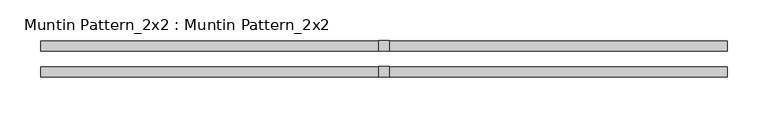
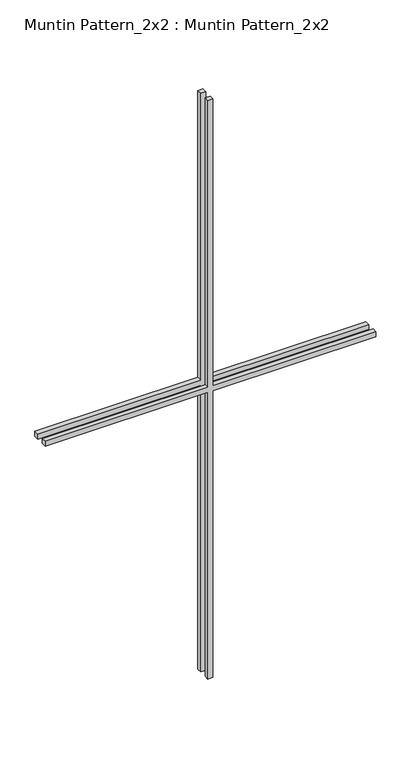
"""IFC4 building model written with IfcOpenShell, lengths in millimetres: proxy geometry, Muntin Pattern_2x2 : Muntin Pattern_2x2."""

import ifcopenshell
import ifcopenshell.guid

model = None  # the IFC model being written
_history = None  # IfcOwnerHistory: only IFC2X3 demands one
_inside = {}  # id of a spatial element -> (the spatial element, [elements in it])
_under = {}  # id of a project, library or spatial element -> (it, [spatial elements below it])
_declared = {}  # id of a project -> (the project, [libraries it declares])
_typed = {}  # id of a type object -> (the type object, [elements of that type])
_made_of = {}  # id of a material, layer set ... -> (it, [elements and type objects made of it])


def new_model(schema):
    """Start an empty IFC model of exactly this schema.

    Asked for "IFC4X3", IfcOpenShell would pick the latest addendum, in which some entities
    have other attributes; the version numbers below select the first issue.
    IFC2X3 requires an IfcOwnerHistory on every rooted entity: one is made here for all.
    """
    global model, _history
    if schema == "IFC4X3":
        model = ifcopenshell.file(schema_version=(4, 3, 0, 0))
    else:
        model = ifcopenshell.file(schema=schema)
    _inside.clear()
    _under.clear()
    _declared.clear()
    _typed.clear()
    _made_of.clear()
    _history = None
    if model.schema == "IFC2X3":
        org = make("IfcOrganization", Name="unknown")
        user = make(
            "IfcPersonAndOrganization",
            ThePerson=make("IfcPerson", FamilyName="unknown"),
            TheOrganization=org,
        )
        app = make(
            "IfcApplication",
            ApplicationDeveloper=org,
            Version="unknown",
            ApplicationFullName="unknown",
            ApplicationIdentifier="unknown",
        )
        _history = make(
            "IfcOwnerHistory",
            OwningUser=user,
            OwningApplication=app,
            ChangeAction="ADDED",
            CreationDate=0,
        )
    return model


def make(cls, **values):
    """One entity of the class cls with the attributes given. An attribute that is None is left unset."""
    return model.create_entity(
        cls, **{name: value for name, value in values.items() if value is not None}
    )


def rooted(cls, **values):
    """An entity with a GlobalId (a new one), such as an element, a storey or a relation."""
    return make(cls, GlobalId=ifcopenshell.guid.new(), OwnerHistory=_history, **values)


def si_unit(unit_type, name, prefix=None):
    """IfcSIUnit, for example si_unit("LENGTHUNIT", "METRE", prefix="MILLI")."""
    return make("IfcSIUnit", UnitType=unit_type, Prefix=prefix, Name=name)


def assignment(units):
    """IfcUnitAssignment: the units of a project."""
    return None if units is None else make("IfcUnitAssignment", Units=units)


def point(xyz):
    """IfcCartesianPoint."""
    return None if xyz is None else make("IfcCartesianPoint", Coordinates=xyz)


def direction(xyz):
    """IfcDirection."""
    return None if xyz is None else make("IfcDirection", DirectionRatios=xyz)


def frame(location, z_axis=None, x_axis=None):
    """IfcAxis2Placement3D, a coordinate frame: its origin and axes. An axis left out is left unset."""
    return make(
        "IfcAxis2Placement3D",
        Location=point(location),
        Axis=direction(z_axis),
        RefDirection=direction(x_axis),
    )


def origin():
    """The frame at (0, 0, 0) with its axes left unset."""
    return frame((0.0, 0.0, 0.0))


def place(relative_to, where):
    """IfcLocalPlacement: puts the frame where relative to a parent placement (None: the world)."""
    return make(
        "IfcLocalPlacement", PlacementRelTo=relative_to, RelativePlacement=where
    )


def context(
    kind, dimensions, precision=None, world=None, true_north=None, identifier=None
):
    """IfcGeometricRepresentationContext, for example the 3D "Model" context."""
    return make(
        "IfcGeometricRepresentationContext",
        ContextIdentifier=identifier,
        ContextType=kind,
        CoordinateSpaceDimension=dimensions,
        Precision=precision,
        WorldCoordinateSystem=world,
        TrueNorth=true_north,
    )


def project(units=None, contexts=None):
    """IfcProject with its units and contexts."""
    return rooted(
        "IfcProject",
        Name="project",
        RepresentationContexts=contexts,
        UnitsInContext=assignment(units),
    )


def spatial(cls, under=None, at=None, **own):
    """A site, building, storey or space (cls), placed at a placement, below another one or the project."""
    s = rooted(cls, ObjectPlacement=at, **own)
    if under is not None:
        _under.setdefault(under.id(), (under, []))[1].append(s)
    return s


def polyline(points):
    """IfcPolyline through the points."""
    return make("IfcPolyline", Points=[point(p) for p in points])


def outline(outer, holes=None, kind="AREA"):
    """IfcArbitraryClosedProfileDef: a profile drawn as a closed curve; with holes, ...WithVoids."""
    if holes is None:
        return make("IfcArbitraryClosedProfileDef", ProfileType=kind, OuterCurve=outer)
    return make(
        "IfcArbitraryProfileDefWithVoids",
        ProfileType=kind,
        OuterCurve=outer,
        InnerCurves=holes,
    )


def extrude(swept, where, along, depth):
    """IfcExtrudedAreaSolid: the profile swept, set in the frame where, extruded along a direction by depth."""
    return make(
        "IfcExtrudedAreaSolid",
        SweptArea=swept,
        Position=where,
        ExtrudedDirection=direction(along),
        Depth=depth,
    )


def shape(context_of_items, identifier, shape_type, items):
    """IfcShapeRepresentation: the items that make up one representation, for example the "Body"."""
    return make(
        "IfcShapeRepresentation",
        ContextOfItems=context_of_items,
        RepresentationIdentifier=identifier,
        RepresentationType=shape_type,
        Items=items,
    )


def source(mapping_origin, context_of_items, identifier, shape_type, items):
    """IfcRepresentationMap: a shape defined once, which mapped items show again and again."""
    return make(
        "IfcRepresentationMap",
        MappingOrigin=mapping_origin,
        MappedRepresentation=shape(context_of_items, identifier, shape_type, items),
    )


def transform(
    local_origin,
    x_axis=None,
    y_axis=None,
    z_axis=None,
    scale=None,
    scale2=None,
    scale3=None,
    uniform=True,
):
    """IfcCartesianTransformationOperator3D, or its non-uniform kind. x_axis, y_axis, z_axis: its Axis1, 2, 3."""
    if uniform:
        return make(
            "IfcCartesianTransformationOperator3D",
            Axis1=direction(x_axis),
            Axis2=direction(y_axis),
            LocalOrigin=point(local_origin),
            Scale=scale,
            Axis3=direction(z_axis),
        )
    return make(
        "IfcCartesianTransformationOperator3DnonUniform",
        Axis1=direction(x_axis),
        Axis2=direction(y_axis),
        LocalOrigin=point(local_origin),
        Scale=scale,
        Axis3=direction(z_axis),
        Scale2=scale2,
        Scale3=scale3,
    )


def mapped(mapping_source, mapping_target):
    """IfcMappedItem: shows the shape of a source again, moved by a transform."""
    return make(
        "IfcMappedItem", MappingSource=mapping_source, MappingTarget=mapping_target
    )


def made_of(thing, what):
    """Note that an element or type object is made of a material, layer set ...; save() writes the relation."""
    if what is not None:
        _made_of.setdefault(what.id(), (what, []))[1].append(thing)
    return thing


def element(
    cls,
    number,
    at=None,
    inside=None,
    cuts=None,
    type_object=None,
    material=None,
    context=None,
    identifier="Body",
    shape_type=None,
    held_by="IfcProductDefinitionShape",
    body=None,
    shapes=None,
    **own,
):
    """One element of the class cls, such as IfcWall. Its Tag is "e" and its number.

    at: its placement. inside: the storey or other place that contains it. cuts: it is an
    opening in that element (IfcRelVoidsElement). A single representation is given by context,
    identifier, shape_type and body (its items); several are given by shapes. held_by: the class
    of the entity that holds the representations. save() writes the other relations.
    """
    e = rooted(cls, Tag="e%d" % number, ObjectPlacement=at, **own)
    if body is not None:
        shapes = [shape(context, identifier, shape_type, body)]
    if shapes is not None:
        e.Representation = make(held_by, Representations=shapes)
    if inside is not None:
        _inside.setdefault(inside.id(), (inside, []))[1].append(e)
    if cuts is not None:
        rooted(
            "IfcRelVoidsElement", RelatingBuildingElement=cuts, RelatedOpeningElement=e
        )
    if type_object is not None:
        _typed.setdefault(type_object.id(), (type_object, []))[1].append(e)
    return made_of(e, material)


def aggregate(whole, parts):
    """IfcRelAggregates: a whole, such as a stair, and the parts it consists of."""
    return rooted("IfcRelAggregates", RelatingObject=whole, RelatedObjects=parts)


def save(model, path):
    """Write the relations noted so far, then the file.

    IfcRelAggregates (storeys below a building ...), IfcRelContainedInSpatialStructure (elements
    in a storey), IfcRelDefinesByType, IfcRelAssociatesMaterial and IfcRelDeclares: one each for
    every whole, place, type object, material and project.
    """
    for whole, parts in _under.values():
        aggregate(whole, parts)
    for where, things in _inside.values():
        rooted(
            "IfcRelContainedInSpatialStructure",
            RelatedElements=things,
            RelatingStructure=where,
        )
    for kind, things in _typed.values():
        rooted("IfcRelDefinesByType", RelatedObjects=things, RelatingType=kind)
    for what, things in _made_of.values():
        rooted("IfcRelAssociatesMaterial", RelatedObjects=things, RelatingMaterial=what)
    for by, libraries in _declared.values():
        rooted("IfcRelDeclares", RelatingContext=by, RelatedDefinitions=libraries)
    model.write(path)


def muntin_pattern_2x2_muntin_pattern_2x2_e2a5a0f5(model_context):
    return source(origin(), model_context, "Body", "SweptSolid", [
        extrude(outline(polyline([(781.05, -6.35), (781.05, -419.1), (768.35, -419.1), (768.35, -6.35), (0.0, -6.35), (0.0, 6.35), (768.35, 6.35), (768.35, 419.1), (781.05, 419.1), (781.05, 6.35), (1549.4, 6.35), (1549.4, -6.35), (781.05, -6.35)])), frame((0.0, 9.525, 0.0), z_axis=(0.0, 1.0, 0.0), x_axis=(0.0, 0.0, 1.0)), (0.0, 0.0, 1.0), 12.7),
        extrude(outline(polyline([(781.05, -6.35), (781.05, -419.1), (768.35, -419.1), (768.35, -6.35), (0.0, -6.35), (0.0, 6.35), (768.35, 6.35), (768.35, 419.1), (781.05, 419.1), (781.05, 6.35), (1549.4, 6.35), (1549.4, -6.35), (781.05, -6.35)])), frame((0.0, -22.225, 0.0), z_axis=(0.0, 1.0, 0.0), x_axis=(0.0, 0.0, 1.0)), (0.0, 0.0, 1.0), 12.7),
    ])


if __name__ == "__main__":
    model = new_model("IFC4")
    model_context = context("Model", 3, world=origin())
    ifc_project = project(units=[si_unit("LENGTHUNIT", "METRE", prefix="MILLI")], contexts=[model_context])
    site = spatial("IfcSite", under=ifc_project)
    building = spatial("IfcBuilding", under=site)
    placement = place(None, origin())
    muntin_pattern_2x2_muntin_pattern_2x2_shape = muntin_pattern_2x2_muntin_pattern_2x2_e2a5a0f5(model_context)
    element("IfcBuildingElementProxy", 1, Name="Muntin Pattern_2x2 : Muntin Pattern_2x2", ObjectType="Muntin Pattern_2x2 : Muntin Pattern_2x2", at=placement, inside=building, context=model_context, shape_type="MappedRepresentation", body=[
        mapped(muntin_pattern_2x2_muntin_pattern_2x2_shape, transform((0.0, 0.0, 0.0), x_axis=(1.0, 0.0, 0.0), y_axis=(0.0, 1.0, 0.0), z_axis=(0.0, 0.0, 1.0))),
    ])
    save(model, "model.ifc")

# Revit data of these elements
# Type "Muntin Pattern_2x2 : Muntin Pattern_2x2"
#   Width [instance default] = 4' - 0"
#   Thickness = 0' - 0 1/2"
#   Height [instance default] = 4' - 0"
#   Distance = 0' - 0 3/4"
#   Interior Material [instance default] = none
#   Exterior Material [instance default] = none
#   Default Elevation = 0
# Element 1 (IfcBuildingElementProxy, "Muntin Pattern_2x2 : Muntin Pattern_2x2")
#   Width = 2' - 9"
#   Height = 5' - 1"
#   Interior Material = Wood - Stained
#   Exterior Material = Clad - White
#   Materials on its faces: "Clad - White", "Wood - Stained"
# Materials
#   "Clad - White": class "Wood", colour RGB 242 242 238, transparency 0, Cost = 0
#   "Wood - Stained": class "Wood", colour RGB 224 178 126, transparency 0, Cost = 0
